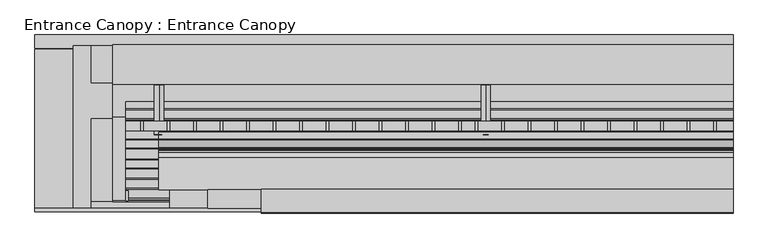
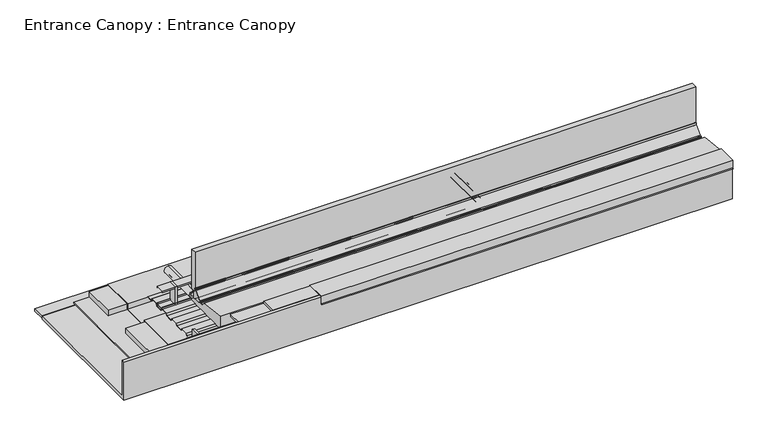
"""IFC4 building model written with IfcOpenShell, lengths in millimetres: proxy geometry, Entrance Canopy : Entrance Canopy."""

from ifc_helpers import new_model, si_unit, point, frame, frame_2d, origin, place, context, project, spatial, polyline, circle_curve, trimmed, segment, composite_curve, outline, extrude, source, transform, mapped, element, save
from ifc_brep_helpers import cylinder_surface, revolved_surface, advanced_brep


def entrance_canopy_entrance_canopy_0983c7dc(model_context):
    return source(origin(), model_context, "Body", "SolidModel", [
        extrude(outline(polyline([(12337.5349983, -311.15), (12337.5349983, -463.55), (12299.4349983, -463.55), (12299.4349983, -311.15), (12337.5349983, -311.15)])), frame((0.0, 0.0, -544.5308974), z_axis=(0.0, 0.0, 1.0), x_axis=(1.0, 0.0, 0.0)), (0.0, 0.0, 1.0), 341.3308974),
        extrude(outline(polyline([(11931.1349983, -311.15), (11931.1349983, -463.55), (11893.0349983, -463.55), (11893.0349983, -311.15), (11931.1349983, -311.15)])), frame((0.0, 0.0, -544.5308974), z_axis=(0.0, 0.0, 1.0), x_axis=(1.0, 0.0, 0.0)), (0.0, 0.0, 1.0), 341.3308974),
        extrude(outline(polyline([(11524.7349983, -311.15), (11524.7349983, -463.55), (11486.6349983, -463.55), (11486.6349983, -311.15), (11524.7349983, -311.15)])), frame((0.0, 0.0, -544.5308974), z_axis=(0.0, 0.0, 1.0), x_axis=(1.0, 0.0, 0.0)), (0.0, 0.0, 1.0), 341.3308974),
        extrude(outline(polyline([(11118.3349983, -311.15), (11118.3349983, -463.55), (11080.2349983, -463.55), (11080.2349983, -311.15), (11118.3349983, -311.15)])), frame((0.0, 0.0, -544.5308974), z_axis=(0.0, 0.0, 1.0), x_axis=(1.0, 0.0, 0.0)), (0.0, 0.0, 1.0), 341.3308974),
        extrude(outline(polyline([(10711.9349983, -311.15), (10711.9349983, -463.55), (10673.8349983, -463.55), (10673.8349983, -311.15), (10711.9349983, -311.15)])), frame((0.0, 0.0, -544.5308974), z_axis=(0.0, 0.0, 1.0), x_axis=(1.0, 0.0, 0.0)), (0.0, 0.0, 1.0), 341.3308974),
        extrude(outline(polyline([(10305.5349983, -311.15), (10305.5349983, -463.55), (10267.4349983, -463.55), (10267.4349983, -311.15), (10305.5349983, -311.15)])), frame((0.0, 0.0, -544.5308974), z_axis=(0.0, 0.0, 1.0), x_axis=(1.0, 0.0, 0.0)), (0.0, 0.0, 1.0), 341.3308974),
        extrude(outline(polyline([(9899.1349983, -311.15), (9899.1349983, -463.55), (9861.0349983, -463.55), (9861.0349983, -311.15), (9899.1349983, -311.15)])), frame((0.0, 0.0, -544.5308974), z_axis=(0.0, 0.0, 1.0), x_axis=(1.0, 0.0, 0.0)), (0.0, 0.0, 1.0), 341.3308974),
        extrude(outline(polyline([(9492.7349983, -311.15), (9492.7349983, -463.55), (9454.6349983, -463.55), (9454.6349983, -311.15), (9492.7349983, -311.15)])), frame((0.0, 0.0, -544.5308974), z_axis=(0.0, 0.0, 1.0), x_axis=(1.0, 0.0, 0.0)), (0.0, 0.0, 1.0), 341.3308974),
        extrude(outline(polyline([(8679.9349983, -311.15), (8679.9349983, -463.55), (8641.8349983, -463.55), (8641.8349983, -311.15), (8679.9349983, -311.15)])), frame((0.0, 0.0, -544.5308974), z_axis=(0.0, 0.0, 1.0), x_axis=(1.0, 0.0, 0.0)), (0.0, 0.0, 1.0), 341.3308974),
        extrude(outline(polyline([(9086.3349983, -311.15), (9086.3349983, -463.55), (9048.2349983, -463.55), (9048.2349983, -311.15), (9086.3349983, -311.15)])), frame((0.0, 0.0, -544.5308974), z_axis=(0.0, 0.0, 1.0), x_axis=(1.0, 0.0, 0.0)), (0.0, 0.0, 1.0), 341.3308974),
        extrude(outline(polyline([(8679.9349983, -311.15), (8679.9349983, -463.55), (8641.8349983, -463.55), (8641.8349983, -311.15), (8679.9349983, -311.15)])), frame((0.0, 0.0, -544.5308974), z_axis=(0.0, 0.0, 1.0), x_axis=(1.0, 0.0, 0.0)), (0.0, 0.0, 1.0), 341.3308974),
        extrude(outline(polyline([(8425.9349983, -311.15), (8425.9349983, -463.55), (8387.8349983, -463.55), (8387.8349983, -311.15), (8425.9349983, -311.15)])), frame((0.0, 0.0, -544.5308974), z_axis=(0.0, 0.0, 1.0), x_axis=(1.0, 0.0, 0.0)), (0.0, 0.0, 1.0), 341.3308974),
        extrude(outline(polyline([(8019.5349983, -311.15), (8019.5349983, -463.55), (7981.4349983, -463.55), (7981.4349983, -311.15), (8019.5349983, -311.15)])), frame((0.0, 0.0, -544.5308974), z_axis=(0.0, 0.0, 1.0), x_axis=(1.0, 0.0, 0.0)), (0.0, 0.0, 1.0), 341.3308974),
        extrude(outline(polyline([(7613.1349983, -311.15), (7613.1349983, -463.55), (7575.0349983, -463.55), (7575.0349983, -311.15), (7613.1349983, -311.15)])), frame((0.0, 0.0, -544.5308974), z_axis=(0.0, 0.0, 1.0), x_axis=(1.0, 0.0, 0.0)), (0.0, 0.0, 1.0), 341.3308974),
        extrude(outline(polyline([(7206.7349983, -311.15), (7206.7349983, -463.55), (7168.6349983, -463.55), (7168.6349983, -311.15), (7206.7349983, -311.15)])), frame((0.0, 0.0, -544.5308974), z_axis=(0.0, 0.0, 1.0), x_axis=(1.0, 0.0, 0.0)), (0.0, 0.0, 1.0), 341.3308974),
        extrude(outline(polyline([(6800.3349983, -311.15), (6800.3349983, -463.55), (6762.2349983, -463.55), (6762.2349983, -311.15), (6800.3349983, -311.15)])), frame((0.0, 0.0, -544.5308974), z_axis=(0.0, 0.0, 1.0), x_axis=(1.0, 0.0, 0.0)), (0.0, 0.0, 1.0), 341.3308974),
        extrude(outline(polyline([(6393.9349983, -311.15), (6393.9349983, -463.55), (6355.8349983, -463.55), (6355.8349983, -311.15), (6393.9349983, -311.15)])), frame((0.0, 0.0, -544.5308974), z_axis=(0.0, 0.0, 1.0), x_axis=(1.0, 0.0, 0.0)), (0.0, 0.0, 1.0), 341.3308974),
        extrude(outline(polyline([(5987.5349983, -311.15), (5987.5349983, -463.55), (5949.4349983, -463.55), (5949.4349983, -311.15), (5987.5349983, -311.15)])), frame((0.0, 0.0, -544.5308974), z_axis=(0.0, 0.0, 1.0), x_axis=(1.0, 0.0, 0.0)), (0.0, 0.0, 1.0), 341.3308974),
        extrude(outline(polyline([(5581.1349983, -311.15), (5581.1349983, -463.55), (5543.0349983, -463.55), (5543.0349983, -311.15), (5581.1349983, -311.15)])), frame((0.0, 0.0, -544.5308974), z_axis=(0.0, 0.0, 1.0), x_axis=(1.0, 0.0, 0.0)), (0.0, 0.0, 1.0), 341.3308974),
        extrude(outline(polyline([(5174.7349983, -311.15), (5174.7349983, -463.55), (5136.6349983, -463.55), (5136.6349983, -311.15), (5174.7349983, -311.15)])), frame((0.0, 0.0, -544.5308974), z_axis=(0.0, 0.0, 1.0), x_axis=(1.0, 0.0, 0.0)), (0.0, 0.0, 1.0), 341.3308974),
        extrude(outline(polyline([(4768.3349983, -311.15), (4768.3349983, -463.55), (4730.2349983, -463.55), (4730.2349983, -311.15), (4768.3349983, -311.15)])), frame((0.0, 0.0, -544.5308974), z_axis=(0.0, 0.0, 1.0), x_axis=(1.0, 0.0, 0.0)), (0.0, 0.0, 1.0), 341.3308974),
        extrude(outline(polyline([(4361.9349983, -311.15), (4361.9349983, -463.55), (4323.8349983, -463.55), (4323.8349983, -311.15), (4361.9349983, -311.15)])), frame((0.0, 0.0, -544.5308974), z_axis=(0.0, 0.0, 1.0), x_axis=(1.0, 0.0, 0.0)), (0.0, 0.0, 1.0), 341.3308974),
        extrude(outline(polyline([(3955.5349983, -311.15), (3955.5349983, -463.55), (3917.4349983, -463.55), (3917.4349983, -311.15), (3955.5349983, -311.15)])), frame((0.0, 0.0, -544.5308974), z_axis=(0.0, 0.0, 1.0), x_axis=(1.0, 0.0, 0.0)), (0.0, 0.0, 1.0), 341.3308974),
        advanced_brep(
        [(8804.275, 238.0930709, -452.4507493), (8804.275, 239.0190623, -363.5555721), (8804.275, -522.9395999, -355.6185027), (8804.275, -523.8655913, -444.5136799), (8804.275, 237.5639329, -477.8466155), (8804.275, 239.0190623, -338.1541941), (8804.275, -524.3947293, -469.9095461), (8804.275, -522.9395999, -330.2171247)],
        [
            (0, 1, circle_curve(frame((8804.275, 238.5560666, -408.0031607), z_axis=(0.0, 0.9999457509425376, -0.010416101572322716), x_axis=(0.0, 0.010416101572322716, 0.9999457509425376)), 44.45)),
            (1, 2),
            (2, 3, circle_curve(frame((8804.275, -523.4025956, -400.0660913), z_axis=(0.0, -0.9999457509425376, 0.010416101572322716), x_axis=(0.0, 0.010416101572322716, 0.9999457509425376)), 44.45)),
            (3, 0),
            (1, 0, circle_curve(frame((8804.275, 238.5560666, -408.0031607), z_axis=(0.0, 0.9999457509425376, -0.010416101572322716), x_axis=(0.0, 0.010416101572322716, 0.9999457509425376)), 44.45)),
            (3, 2, circle_curve(frame((8804.275, -523.4025956, -400.0660913), z_axis=(0.0, -0.9999457509425376, 0.010416101572322716), x_axis=(0.0, 0.010416101572322716, 0.9999457509425376)), 44.45)),
            (4, 5, circle_curve(frame((8804.275, 238.2914976, -408.0004048), z_axis=(0.0, 0.9999457509425376, -0.010416101572322716), x_axis=(0.0, 0.010416101572322716, 0.9999457509425376)), 69.85)),
            (5, 1),
            (0, 4),
            (5, 4, circle_curve(frame((8804.275, 238.2914976, -408.0004048), z_axis=(0.0, 0.9999457509425376, -0.010416101572322716), x_axis=(0.0, 0.010416101572322716, 0.9999457509425376)), 69.85)),
            (6, 7, circle_curve(frame((8804.275, -523.6671646, -400.0633354), z_axis=(0.0, 0.9999457509425376, -0.010416101572322716), x_axis=(0.0, 0.010416101572322716, 0.9999457509425376)), 69.85)),
            (7, 5),
            (4, 6),
            (7, 6, circle_curve(frame((8804.275, -523.6671646, -400.0633354), z_axis=(0.0, 0.9999457509425376, -0.010416101572322716), x_axis=(0.0, 0.010416101572322716, 0.9999457509425376)), 69.85)),
            (2, 7),
            (6, 3),
        ],
        [
            revolved_surface(polyline([(8804.275, -522.939599899714, -355.6185026725319), (8804.275, 239.0190623294717, -363.5555720707561)]), (8804.275, 238.5560666, -408.0031607), (0.0, -0.9999457509425376, 0.010416101572322716)),
            revolved_surface(polyline([(8804.275, 239.0190623, -363.5555721), (8804.275, 239.0190623, -338.1541941)]), (8804.275, 238.5560666, -408.0031607), (0.0, -0.9999457509425376, 0.010416101572322716)),
            cylinder_surface(frame((8804.275, 238.5560666, -408.0031607), z_axis=(0.0, -0.9999457509425376, 0.010416101572322716), x_axis=(0.0, 0.010416101572322716, 0.9999457509425376)), 69.85),
            revolved_surface(polyline([(8804.275, -522.9395999, -330.2171247), (8804.275, -522.9395999, -355.6185027)]), (8804.275, 238.5560666, -408.0031607), (0.0, -0.9999457509425376, 0.010416101572322716)),
        ],
        [
            (0, [[1, 2, 3, 4]]),
            (0, [[5, -4, 6, -2]]),
            (1, [[7, 8, -1, 9]]),
            (1, [[10, -9, -5, -8]]),
            (2, [[11, 12, -7, 13]]),
            (2, [[14, -13, -10, -12]]),
            (3, [[-3, 15, -11, 16]]),
            (3, [[-6, -16, -14, -15]]),
        ],
    ),
        advanced_brep(
        [(3794.125, 238.0930709, -452.4507493), (3794.125, 239.0190623, -363.5555721), (3794.125, -522.9395999, -355.6185027), (3794.125, -523.8655913, -444.5136799), (3794.125, 237.5639329, -477.8466155), (3794.125, 239.0190623, -338.1541941), (3794.125, -524.3947293, -469.9095461), (3794.125, -522.9395999, -330.2171247)],
        [
            (0, 1, circle_curve(frame((3794.125, 238.5560666, -408.0031607), z_axis=(0.0, 0.9999457509425376, -0.010416101572322716), x_axis=(0.0, 0.010416101572322716, 0.9999457509425376)), 44.45)),
            (1, 2),
            (2, 3, circle_curve(frame((3794.125, -523.4025956, -400.0660913), z_axis=(0.0, -0.9999457509425376, 0.010416101572322716), x_axis=(0.0, 0.010416101572322716, 0.9999457509425376)), 44.45)),
            (3, 0),
            (1, 0, circle_curve(frame((3794.125, 238.5560666, -408.0031607), z_axis=(0.0, 0.9999457509425376, -0.010416101572322716), x_axis=(0.0, 0.010416101572322716, 0.9999457509425376)), 44.45)),
            (3, 2, circle_curve(frame((3794.125, -523.4025956, -400.0660913), z_axis=(0.0, -0.9999457509425376, 0.010416101572322716), x_axis=(0.0, 0.010416101572322716, 0.9999457509425376)), 44.45)),
            (4, 5, circle_curve(frame((3794.125, 238.2914976, -408.0004048), z_axis=(0.0, 0.9999457509425376, -0.010416101572322716), x_axis=(0.0, 0.010416101572322716, 0.9999457509425376)), 69.85)),
            (5, 1),
            (0, 4),
            (5, 4, circle_curve(frame((3794.125, 238.2914976, -408.0004048), z_axis=(0.0, 0.9999457509425376, -0.010416101572322716), x_axis=(0.0, 0.010416101572322716, 0.9999457509425376)), 69.85)),
            (6, 7, circle_curve(frame((3794.125, -523.6671646, -400.0633354), z_axis=(0.0, 0.9999457509425376, -0.010416101572322716), x_axis=(0.0, 0.010416101572322716, 0.9999457509425376)), 69.85)),
            (7, 5),
            (4, 6),
            (7, 6, circle_curve(frame((3794.125, -523.6671646, -400.0633354), z_axis=(0.0, 0.9999457509425376, -0.010416101572322716), x_axis=(0.0, 0.010416101572322716, 0.9999457509425376)), 69.85)),
            (2, 7),
            (6, 3),
        ],
        [
            revolved_surface(polyline([(3794.125, -522.939599899714, -355.6185026725319), (3794.125, 239.0190623294717, -363.5555720707561)]), (3794.125, 238.5560666, -408.0031607), (0.0, -0.9999457509425376, 0.010416101572322716)),
            revolved_surface(polyline([(3794.125, 239.0190623, -363.5555721), (3794.125, 239.0190623, -338.1541941)]), (3794.125, 238.5560666, -408.0031607), (0.0, -0.9999457509425376, 0.010416101572322716)),
            cylinder_surface(frame((3794.125, 238.5560666, -408.0031607), z_axis=(0.0, -0.9999457509425376, 0.010416101572322716), x_axis=(0.0, 0.010416101572322716, 0.9999457509425376)), 69.85),
            revolved_surface(polyline([(3794.125, -522.9395999, -330.2171247), (3794.125, -522.9395999, -355.6185027)]), (3794.125, 238.5560666, -408.0031607), (0.0, -0.9999457509425376, 0.010416101572322716)),
        ],
        [
            (0, [[1, 2, 3, 4]]),
            (0, [[5, -4, 6, -2]]),
            (1, [[7, 8, -1, 9]]),
            (1, [[10, -9, -5, -8]]),
            (2, [[11, 12, -7, 13]]),
            (2, [[14, -13, -10, -12]]),
            (3, [[-3, 15, -11, 16]]),
            (3, [[-6, -16, -14, -15]]),
        ],
    ),
        extrude(outline(polyline([(-1365.25, -297.0477336), (-1365.25, -285.75), (-1701.8, -285.75), (-1701.8, -425.238552), (-1722.3378953, -425.238552), (-1709.6378953, -412.538552), (-1709.6378953, -272.838552), (-1357.9881919, -279.8500104), (-1357.9881919, -297.0477336), (-1365.25, -297.0477336)])), frame((5360.5622491, 0.0, 0.0), z_axis=(1.0, 0.0, 0.0), x_axis=(0.0, 1.0, 0.0)), (0.0, 0.0, 1.0), 7237.8377509),
        advanced_brep(
        [(8804.275, -522.9395999, -355.6185027), (8804.275, -523.8655913, -444.5136799), (8804.275, 238.0930709, -452.4507493), (8804.275, 239.0190623, -363.5555721), (8804.275, 238.0930709, -407.9983378), (8804.275, -523.8655913, -400.0612684)],
        [
            (0, 1, circle_curve(frame((8804.275, -523.4025956, -400.0660913), z_axis=(0.0, 0.9999457509425375, -0.010416101572321135), x_axis=(0.0, -0.010416101572321135, -0.9999457509425375)), 44.45)),
            (1, 2),
            (2, 3, circle_curve(frame((8804.275, 238.5560666, -408.0031607), z_axis=(0.0, -0.9999457509425375, 0.010416101572321135), x_axis=(0.0, -0.010416101572321135, -0.9999457509425375)), 44.45)),
            (3, 0),
            (1, 0, circle_curve(frame((8804.275, -523.4025956, -400.0660913), z_axis=(0.0, 0.9999457509425375, -0.010416101572321135), x_axis=(0.0, -0.010416101572321135, -0.9999457509425375)), 44.45)),
            (3, 2, circle_curve(frame((8804.275, 238.5560666, -408.0031607), z_axis=(0.0, -0.9999457509425375, 0.010416101572321135), x_axis=(0.0, -0.010416101572321135, -0.9999457509425375)), 44.45)),
            (2, 4),
            (4, 3),
            (5, 1),
            (0, 5),
        ],
        [
            cylinder_surface(frame((8804.275, -112.5209117, -404.3461088), z_axis=(0.0, -0.9999457509425375, 0.010416101572321135), x_axis=(0.0, -0.010416101572321135, -0.9999457509425375)), 44.45),
            revolved_surface(polyline([(8804.275, 238.0930709, -407.9983378), (8804.275, 238.0930709, -452.4507493)]), (8804.275, -112.5209117, -404.3461088), (0.0, -0.9999457509425375, 0.010416101572321135)),
            revolved_surface(polyline([(8804.275, -523.8655913, -444.5136799), (8804.275, -523.8655913, -400.0612684)]), (8804.275, -112.5209117, -404.3461088), (0.0, -0.9999457509425375, 0.010416101572321135)),
        ],
        [
            (0, [[1, 2, 3, 4]]),
            (0, [[5, -4, 6, -2]]),
            (1, [[-3, 7, 8]]),
            (1, [[-6, -8, -7]]),
            (2, [[9, -1, 10]]),
            (2, [[-10, -5, -9]]),
        ],
    ),
        advanced_brep(
        [(3794.125, 239.0190623, -363.5555721), (3794.125, 238.0930709, -452.4507493), (3794.125, -523.8655913, -444.5136799), (3794.125, -522.9395999, -355.6185027), (3794.125, 238.0930709, -407.9983378), (3794.125, -523.8655913, -400.0612684)],
        [
            (0, 1, circle_curve(frame((3794.125, 238.5560666, -408.0031607), z_axis=(0.0, -0.9999457509425375, 0.010416101572321135), x_axis=(0.0, -0.010416101572321135, -0.9999457509425375)), 44.45)),
            (1, 2),
            (2, 3, circle_curve(frame((3794.125, -523.4025956, -400.0660913), z_axis=(0.0, 0.9999457509425375, -0.010416101572321135), x_axis=(0.0, -0.010416101572321135, -0.9999457509425375)), 44.45)),
            (3, 0),
            (1, 0, circle_curve(frame((3794.125, 238.5560666, -408.0031607), z_axis=(0.0, -0.9999457509425375, 0.010416101572321135), x_axis=(0.0, -0.010416101572321135, -0.9999457509425375)), 44.45)),
            (3, 2, circle_curve(frame((3794.125, -523.4025956, -400.0660913), z_axis=(0.0, 0.9999457509425375, -0.010416101572321135), x_axis=(0.0, -0.010416101572321135, -0.9999457509425375)), 44.45)),
            (4, 1),
            (0, 4),
            (2, 5),
            (5, 3),
        ],
        [
            cylinder_surface(frame((3794.125, -112.5209117, -404.3461088), z_axis=(0.0, 0.9999457509425375, -0.010416101572321135), x_axis=(0.0, -0.010416101572321135, -0.9999457509425375)), 44.45),
            revolved_surface(polyline([(3794.125, 238.0930709, -452.4507493), (3794.125, 238.0930709, -407.9983378)]), (3794.125, -112.5209117, -404.3461088), (0.0, 0.9999457509425375, -0.010416101572321135)),
            revolved_surface(polyline([(3794.125, -523.8655913, -400.0612684), (3794.125, -523.8655913, -444.5136799)]), (3794.125, -112.5209117, -404.3461088), (0.0, 0.9999457509425375, -0.010416101572321135)),
        ],
        [
            (0, [[1, 2, 3, 4]]),
            (0, [[5, -4, 6, -2]]),
            (1, [[7, -1, 8]]),
            (1, [[-8, -5, -7]]),
            (2, [[-3, 9, 10]]),
            (2, [[-6, -10, -9]]),
        ],
    ),
        extrude(outline(composite_curve([segment(polyline([(-523.8655913, -332.7816197), (-523.8655913, -462.9741541), (-561.8697705, -462.9741541)]), True, "CONTINUOUS"), segment(trimmed(circle_curve(frame_2d((-577.3448907, -474.0881509)), 19.052566), [point((-561.8697705, -462.9741541))], [point((-577.3448907, -455.0355849))], True, "CARTESIAN"), True, "CONTINUOUS"), segment(polyline([(-577.3448907, -455.0355849), (-689.2602386, -455.0355849)]), True, "CONTINUOUS"), segment(trimmed(circle_curve(frame_2d((-689.2602386, -445.5093019)), 9.526283), [point((-689.2602386, -455.0355849))], [point((-695.9963379, -452.2454012))], False, "CARTESIAN"), True, "CONTINUOUS"), segment(polyline([(-695.9963379, -452.2454012), (-722.4426559, -425.7990833)]), True, "CONTINUOUS"), segment(trimmed(circle_curve(frame_2d((-724.6880223, -428.0444497)), 3.1754277), [point((-722.4426559, -425.7990833))], [point((-724.6880223, -424.8690221))], True, "CARTESIAN"), True, "CONTINUOUS"), segment(polyline([(-724.6880223, -424.8690221), (-728.6806758, -424.8690221)]), True, "CONTINUOUS"), segment(trimmed(circle_curve(frame_2d((-728.6806758, -428.0444497)), 3.1754277), [point((-728.6806758, -424.8690221))], [point((-731.8561035, -428.0444497))], True, "CARTESIAN"), True, "CONTINUOUS"), segment(polyline([(-731.8561035, -428.0444497), (-731.8561035, -435.9830189)]), True, "CONTINUOUS"), segment(trimmed(circle_curve(frame_2d((-735.0315312, -435.9830189)), 3.1754277), [point((-731.8561035, -435.9830189))], [point((-735.0315312, -439.1584466))], False, "CARTESIAN"), True, "CONTINUOUS"), segment(polyline([(-735.0315312, -439.1584466), (-744.5578142, -439.1584466)]), True, "CONTINUOUS"), segment(trimmed(circle_curve(frame_2d((-744.5578142, -435.9830189)), 3.1754277), [point((-744.5578142, -439.1584466))], [point((-747.7332419, -435.9830189))], False, "CARTESIAN"), True, "CONTINUOUS"), segment(polyline([(-747.7332419, -435.9830189), (-747.7332419, -428.0444497)]), True, "CONTINUOUS"), segment(trimmed(circle_curve(frame_2d((-750.9086695, -428.0444497)), 3.1754277), [point((-747.7332419, -428.0444497))], [point((-750.9086695, -424.8690221))], True, "CARTESIAN"), True, "CONTINUOUS"), segment(polyline([(-750.9086695, -424.8690221), (-754.0840972, -424.8690221)]), True, "CONTINUOUS"), segment(trimmed(circle_curve(frame_2d((-754.0840972, -423.2813082)), 1.5877138), [point((-754.0840972, -424.8690221))], [point((-755.671811, -423.2813082))], False, "CARTESIAN"), True, "CONTINUOUS"), segment(polyline([(-755.671811, -423.2813082), (-755.671811, -410.5795976), (-719.9482498, -410.5795976), (-600.0758553, -289.1194893), (-600.0758553, -254.9836419), (-593.725, -254.9836419), (-587.3741447, -254.9836419)]), True, "CONTINUOUS"), segment(trimmed(circle_curve(frame_2d((-587.3741447, -256.5713557)), 1.5877138), [point((-587.3741447, -254.9836419))], [point((-585.7864308, -256.5713557))], False, "CARTESIAN"), True, "CONTINUOUS"), segment(polyline([(-585.7864308, -256.5713557), (-585.7864308, -259.7467834)]), True, "CONTINUOUS"), segment(trimmed(circle_curve(frame_2d((-582.6110032, -259.7467834)), 3.1754277), [point((-585.7864308, -259.7467834))], [point((-582.6110032, -262.9222111))], True, "CARTESIAN"), True, "CONTINUOUS"), segment(polyline([(-582.6110032, -262.9222111), (-574.672434, -262.9222111)]), True, "CONTINUOUS"), segment(trimmed(circle_curve(frame_2d((-574.672434, -266.0976387)), 3.1754277), [point((-574.672434, -262.9222111))], [point((-571.4970063, -266.0976387))], False, "CARTESIAN"), True, "CONTINUOUS"), segment(polyline([(-571.4970063, -266.0976387), (-571.4970063, -275.6239217)]), True, "CONTINUOUS"), segment(trimmed(circle_curve(frame_2d((-574.672434, -275.6239217)), 3.1754277), [point((-571.4970063, -275.6239217))], [point((-574.672434, -278.7993494))], False, "CARTESIAN"), True, "CONTINUOUS"), segment(polyline([(-574.672434, -278.7993494), (-582.6110032, -278.7993494)]), True, "CONTINUOUS"), segment(trimmed(circle_curve(frame_2d((-582.6110032, -281.9747771)), 3.1754277), [point((-582.6110032, -278.7993494))], [point((-585.7864308, -281.9747771))], True, "CARTESIAN"), True, "CONTINUOUS"), segment(polyline([(-585.7864308, -281.9747771), (-585.7864308, -285.9674306)]), True, "CONTINUOUS"), segment(trimmed(circle_curve(frame_2d((-582.6110032, -285.9674306)), 3.1754277), [point((-585.7864308, -285.9674306))], [point((-584.8563696, -288.212797))], True, "CARTESIAN"), True, "CONTINUOUS"), segment(polyline([(-584.8563696, -288.212797), (-557.4799905, -315.5891762)]), True, "CONTINUOUS"), segment(trimmed(circle_curve(frame_2d((-561.9707233, -320.0799091)), 6.3508553), [point((-557.4799905, -315.5891762))], [point((-555.619868, -320.0799091))], False, "CARTESIAN"), True, "CONTINUOUS"), segment(polyline([(-555.619868, -320.0799091), (-555.619868, -329.6061921)]), True, "CONTINUOUS"), segment(trimmed(circle_curve(frame_2d((-552.4444403, -329.6061921)), 3.1754277), [point((-555.619868, -329.6061921))], [point((-552.4444403, -332.7816197))], True, "CARTESIAN"), True, "CONTINUOUS"), segment(polyline([(-552.4444403, -332.7816197), (-523.8655913, -332.7816197)]), True, "CONTINUOUS")], self_intersect=False)), frame((3792.8941209, 0.0, 0.0), z_axis=(1.0, 0.0, 0.0), x_axis=(0.0, 1.0, 0.0)), (0.0, 0.0, 1.0), 8805.5058791),
        extrude(outline(polyline([(3549.1349983, -311.15), (3549.1349983, -463.55), (3511.0349983, -463.55), (3511.0349983, -311.15), (3549.1349983, -311.15)])), frame((0.0, 0.0, -544.5308974), z_axis=(0.0, 0.0, 1.0), x_axis=(1.0, 0.0, 0.0)), (0.0, 0.0, 1.0), 341.3308974),
        extrude(outline(polyline([(-312.36412, -509.6058974), (-311.15, -509.6058974), (-311.15, -544.5308974), (-463.55, -544.5308974), (-463.55, -509.6058974), (-462.33588, -509.6058974), (-462.33588, -543.3167774), (-312.36412, -543.3167774), (-312.36412, -509.6058974)])), frame((3282.4349983, 0.0, 0.0), z_axis=(1.0, 0.0, 0.0), x_axis=(0.0, 1.0, 0.0)), (0.0, 0.0, 1.0), 9315.9650017),
        extrude(outline(polyline([(-312.36412, -238.125), (-312.36412, -204.41412), (-462.33588, -204.41412), (-462.33588, -238.125), (-463.55, -238.125), (-463.55, -203.2), (-311.15, -203.2), (-311.15, -238.125), (-312.36412, -238.125)])), frame((3282.4349983, 0.0, 0.0), z_axis=(1.0, 0.0, 0.0), x_axis=(0.0, 1.0, 0.0)), (0.0, 0.0, 1.0), 9315.9650017),
        extrude(outline(polyline([(-295.0199508, -584.2183974), (-423.5043821, -584.2183974), (-443.020825, -546.1183974), (-580.3035079, -546.1183974), (-599.8199508, -584.2183974), (-728.3043821, -584.2183974), (-747.820825, -546.1183974), (-885.1035079, -546.1183974), (-904.6199508, -584.2183974), (-1033.1043821, -584.2183974), (-1052.620825, -546.1183974), (-1189.9035079, -546.1183974), (-1209.4199508, -584.2183974), (-1337.9043821, -584.2183974), (-1357.420825, -546.1183974), (-1494.7035079, -546.1183974), (-1514.2199508, -584.2183974), (-1516.0036062, -584.2183974), (-1495.6739781, -544.5308974), (-1356.4503548, -544.5308974), (-1336.9339119, -582.6308974), (-1210.390421, -582.6308974), (-1190.8739781, -544.5308974), (-1051.6503548, -544.5308974), (-1032.1339119, -582.6308974), (-905.590421, -582.6308974), (-886.0739781, -544.5308974), (-746.8503548, -544.5308974), (-727.3339119, -582.6308974), (-600.790421, -582.6308974), (-581.2739781, -544.5308974), (-442.0503548, -544.5308974), (-422.5339119, -582.6308974), (-295.990421, -582.6308974), (-276.4739781, -544.5308974), (-137.2503548, -544.5308974), (-117.7339119, -582.6308974), (-12.192, -582.6308974), (-12.192, -584.2183974), (-118.7043821, -584.2183974), (-138.220825, -546.1183974), (-275.5035079, -546.1183974), (-295.0199508, -584.2183974)])), frame((3282.4349983, 0.0, 0.0), z_axis=(1.0, 0.0, 0.0), x_axis=(0.0, 1.0, 0.0)), (0.0, 0.0, 1.0), 9315.9650017),
        extrude(outline(composite_curve([segment(polyline([(-1365.25, -304.735136), (-864.2884987, -362.1930859), (-794.7639215, -431.8132654), (-747.7332419, -431.8132654), (-747.7332419, -435.9830189)]), True, "CONTINUOUS"), segment(trimmed(circle_curve(frame_2d((-744.5578142, -435.9830189)), 3.1754277), [point((-747.7332419, -435.9830189))], [point((-744.5578142, -439.1584466))], True, "CARTESIAN"), True, "CONTINUOUS"), segment(polyline([(-744.5578142, -439.1584466), (-735.0315312, -439.1584466)]), True, "CONTINUOUS"), segment(trimmed(circle_curve(frame_2d((-735.0315312, -435.9830189)), 3.1754277), [point((-735.0315312, -439.1584466))], [point((-731.8561035, -435.9830189))], True, "CARTESIAN"), True, "CONTINUOUS"), segment(polyline([(-731.8561035, -435.9830189), (-731.8561035, -428.0444497)]), True, "CONTINUOUS"), segment(trimmed(circle_curve(frame_2d((-728.6806758, -428.0444497)), 3.1754277), [point((-731.8561035, -428.0444497))], [point((-728.6806758, -424.8690221))], False, "CARTESIAN"), True, "CONTINUOUS"), segment(polyline([(-728.6806758, -424.8690221), (-724.6880223, -424.8690221)]), True, "CONTINUOUS"), segment(trimmed(circle_curve(frame_2d((-724.6880223, -428.0444497)), 3.1754277), [point((-724.6880223, -424.8690221))], [point((-722.4426559, -425.7990833))], False, "CARTESIAN"), True, "CONTINUOUS"), segment(polyline([(-722.4426559, -425.7990833), (-695.9963379, -452.2454012)]), True, "CONTINUOUS"), segment(trimmed(circle_curve(frame_2d((-689.2602386, -445.5093019)), 9.526283), [point((-695.9963379, -452.2454012))], [point((-689.2602386, -455.0355849))], True, "CARTESIAN"), True, "CONTINUOUS"), segment(polyline([(-689.2602386, -455.0355849), (-577.3448907, -455.0355849)]), True, "CONTINUOUS"), segment(trimmed(circle_curve(frame_2d((-577.3448907, -474.0881509)), 19.052566), [point((-577.3448907, -455.0355849))], [point((-561.8697705, -462.9741541))], False, "CARTESIAN"), True, "CONTINUOUS"), segment(polyline([(-561.8697705, -462.9741541), (-523.8655913, -462.9741541), (-523.8655913, -332.7816197), (-552.4444403, -332.7816197)]), True, "CONTINUOUS"), segment(trimmed(circle_curve(frame_2d((-552.4444403, -329.6061921)), 3.1754277), [point((-552.4444403, -332.7816197))], [point((-555.619868, -329.6061921))], False, "CARTESIAN"), True, "CONTINUOUS"), segment(polyline([(-555.619868, -329.6061921), (-555.619868, -320.0799091)]), True, "CONTINUOUS"), segment(trimmed(circle_curve(frame_2d((-561.9707233, -320.0799091)), 6.3508553), [point((-555.619868, -320.0799091))], [point((-557.4799905, -315.5891762))], True, "CARTESIAN"), True, "CONTINUOUS"), segment(polyline([(-557.4799905, -315.5891762), (-584.8563696, -288.212797)]), True, "CONTINUOUS"), segment(trimmed(circle_curve(frame_2d((-582.6110032, -285.9674306)), 3.1754277), [point((-584.8563696, -288.212797))], [point((-585.7864308, -285.9674306))], False, "CARTESIAN"), True, "CONTINUOUS"), segment(polyline([(-585.7864308, -285.9674306), (-585.7864308, -281.9747771)]), True, "CONTINUOUS"), segment(trimmed(circle_curve(frame_2d((-582.6110032, -281.9747771)), 3.1754277), [point((-585.7864308, -281.9747771))], [point((-582.6110032, -278.7993494))], False, "CARTESIAN"), True, "CONTINUOUS"), segment(polyline([(-582.6110032, -278.7993494), (-574.672434, -278.7993494)]), True, "CONTINUOUS"), segment(trimmed(circle_curve(frame_2d((-574.672434, -275.6239217)), 3.1754277), [point((-574.672434, -278.7993494))], [point((-571.4970063, -275.6239217))], True, "CARTESIAN"), True, "CONTINUOUS"), segment(polyline([(-571.4970063, -275.6239217), (-571.4970063, -266.0976387)]), True, "CONTINUOUS"), segment(trimmed(circle_curve(frame_2d((-574.672434, -266.0976387)), 3.1754277), [point((-571.4970063, -266.0976387))], [point((-574.672434, -262.9222111))], True, "CARTESIAN"), True, "CONTINUOUS"), segment(polyline([(-574.672434, -262.9222111), (-581.025, -262.9222111), (-581.025, 406.4), (-479.425, 406.4), (-479.425, -544.5308974), (-1365.25, -544.5308974), (-1365.25, -304.735136)]), True, "CONTINUOUS")], self_intersect=False)), frame((3792.8941209, 0.0, 0.0), z_axis=(1.0, 0.0, 0.0), x_axis=(0.0, 1.0, 0.0)), (0.0, 0.0, 1.0), 8805.5058791),
        extrude(outline(polyline([(3323.5325852, -1381.125), (3323.5325852, -1533.525), (3282.4349983, -1533.525), (3282.4349983, -1381.125), (3323.5325852, -1381.125)])), frame((0.0, 0.0, -807.1612), z_axis=(0.0, 0.0, 1.0), x_axis=(1.0, 0.0, 0.0)), (0.0, 0.0, 1.0), 445.2112),
        extrude(outline(polyline([(841.375, -823.0362), (272.48612, -823.0362), (272.48612, -924.6362), (-272.48612, -924.6362), (-272.48612, -823.0362), (-1549.4, -823.0362), (-1549.4, -361.95), (-1533.525, -361.95), (-1533.525, -807.1612), (-256.6113191, -807.1612), (-256.6113191, -907.85188), (256.6112634, -907.85188), (256.6112634, -807.1612), (857.25, -807.1612), (857.25, -942.975), (841.375, -942.975), (841.375, -823.0362)])), frame((3087.6943179, 0.0, 0.0), z_axis=(1.0, 0.0, 0.0), x_axis=(0.0, 1.0, 0.0)), (0.0, 0.0, 1.0), 9510.7056821),
        extrude(outline(polyline([(803.275, -942.975), (803.275, -996.95), (786.4040798, -996.95), (786.4040798, -946.15), (-1651.0, -946.15), (-1651.0, -924.6362), (841.375, -924.6362), (841.375, -942.975), (803.275, -942.975)])), frame((2477.7613839, 0.0, 0.0), z_axis=(1.0, 0.0, 0.0), x_axis=(0.0, 1.0, 0.0)), (0.0, 0.0, 1.0), 10120.6386161),
        extrude(outline(polyline([(12598.4, 1009.65), (12598.4, 803.275), (1890.9304707, 803.275), (1890.9304707, 1009.65), (12598.4, 1009.65)])), frame((0.0, 0.0, -981.075), z_axis=(0.0, 0.0, 1.0), x_axis=(1.0, 0.0, 0.0)), (0.0, 0.0, 1.0), 38.1),
        extrude(outline(polyline([(-1549.4, -823.0362), (-272.48612, -823.0362), (-272.48612, -924.6362), (-1651.0, -924.6362), (-1651.0, -361.95), (-1549.4, -361.95), (-1549.4, -823.0362)])), frame((2752.0100444, 0.0, 0.0), z_axis=(1.0, 0.0, 0.0), x_axis=(0.0, 1.0, 0.0)), (0.0, 0.0, 1.0), 9846.3899556),
        extrude(outline(polyline([(12598.4, 841.375), (12598.4, 272.48612), (2752.0100444, 272.48612), (2752.0100444, 841.375), (12598.4, 841.375)])), frame((0.0, 0.0, -924.6362), z_axis=(0.0, 0.0, 1.0), x_axis=(1.0, 0.0, 0.0)), (0.0, 0.0, 1.0), 101.6),
        extrude(outline(polyline([(12598.4, -1365.25), (12598.4, -1651.0), (3959.9466652, -1651.0), (3959.9466652, -1365.25), (12598.4, -1365.25)])), frame((0.0, 0.0, -361.95), z_axis=(0.0, 0.0, 1.0), x_axis=(1.0, 0.0, 0.0)), (0.0, 0.0, 1.0), 38.1),
        extrude(outline(polyline([(12598.4, -1365.25), (12598.4, -1651.0), (4542.5136019, -1651.0), (4542.5136019, -1365.25), (12598.4, -1365.25)])), frame((0.0, 0.0, -323.85), z_axis=(0.0, 0.0, 1.0), x_axis=(1.0, 0.0, 0.0)), (0.0, 0.0, 1.0), 38.1),
        extrude(outline(polyline([(786.4040798, -946.15), (786.4040798, -996.95), (-1701.8, -996.95), (-1701.8, -285.75), (-1651.0, -285.75), (-1651.0, -946.15), (786.4040798, -946.15)])), frame((1890.9304707, 0.0, 0.0), z_axis=(1.0, 0.0, 0.0), x_axis=(0.0, 1.0, 0.0)), (0.0, 0.0, 1.0), 10707.4695293),
    ])


if __name__ == "__main__":
    model = new_model("IFC4")
    model_context = context("Model", 3, world=origin())
    ifc_project = project(units=[si_unit("LENGTHUNIT", "METRE", prefix="MILLI")], contexts=[model_context])
    site = spatial("IfcSite", under=ifc_project)
    building = spatial("IfcBuilding", under=site)
    placement = place(None, origin())
    entrance_canopy_entrance_canopy_shape = entrance_canopy_entrance_canopy_0983c7dc(model_context)
    element("IfcBuildingElementProxy", 1, Name="Entrance Canopy : Entrance Canopy", ObjectType="Entrance Canopy : Entrance Canopy", at=placement, inside=building, context=model_context, shape_type="MappedRepresentation", body=[
        mapped(entrance_canopy_entrance_canopy_shape, transform((0.0, 0.0, 0.0), x_axis=(1.0, 0.0, 0.0), y_axis=(0.0, 1.0, 0.0), z_axis=(0.0, 0.0, 1.0))),
    ])
    save(model, "model.ifc")

# Revit data of these elements
# Element 1 (IfcBuildingElementProxy, "Entrance Canopy : Entrance Canopy")
#   Materials on its faces: "Stud", "Gutter", "RED", "Orange", "Purple", "Green", "Magenta", "Blue"
# Materials
#   "Stud": class "Generic", colour RGB 64 128 128, transparency 0, Cost = 0
#   "Gutter": class "Generic", colour RGB 128 0 64, transparency 0, Cost = 0
#   "RED": class "Generic", colour RGB 255 0 0, transparency 0, Cost = 0
#   "Orange": class "Generic", colour RGB 255 128 64, transparency 0, Cost = 0
#   "Purple": class "Generic", colour RGB 128 0 255, transparency 0, Cost = 0
#   "Green": class "Generic", colour RGB 0 255 0, transparency 0, Cost = 0
#   "Magenta": class "Generic", colour RGB 255 0 255, transparency 0, Cost = 0
#   "Blue": class "Generic", colour RGB 170 209 217, transparency 0, Cost = 0
